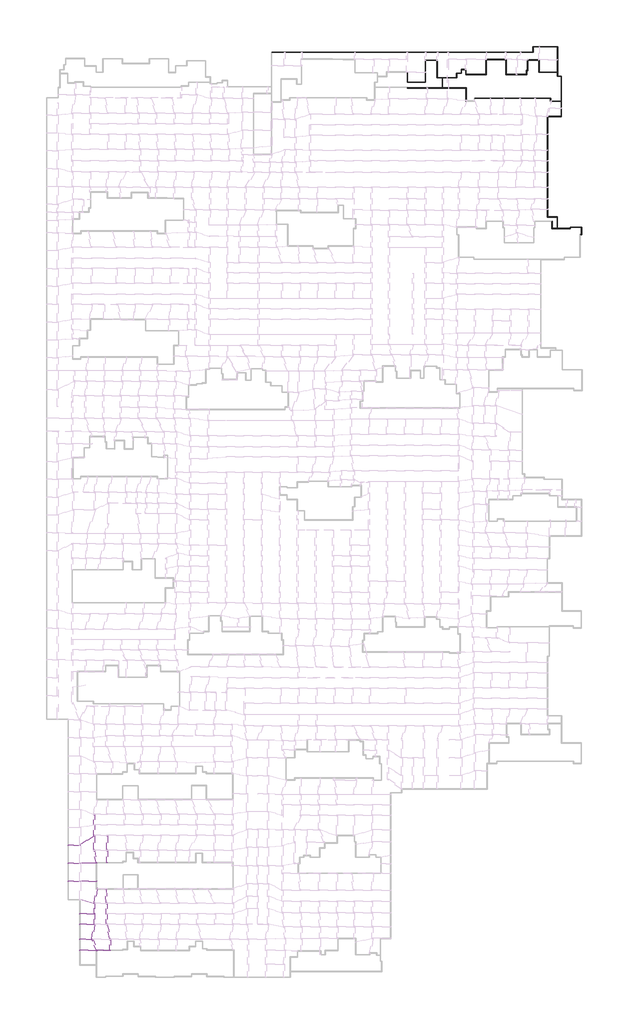
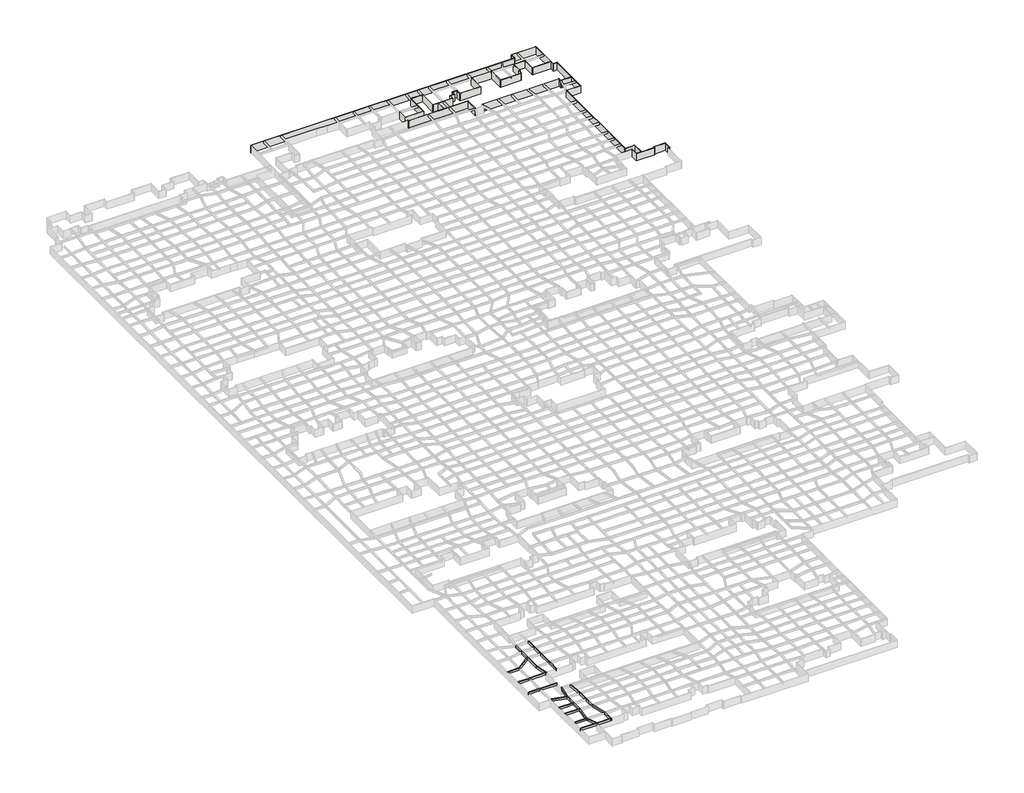
# One storey, part 10 of 45: 45 walls, 24 beams.
"""IFC4 building model written with IfcOpenShell, lengths in millimetres."""

from ifc_helpers import new_model, si_unit, frame, origin, origin_with_axes, place, context, project, spatial, polyline, outline, extrude, faceted_brep, element, save

model = new_model("IFC4")

# Units and contexts
model_context = context("Model", 3, world=origin())
ifc_project = project(units=[si_unit("LENGTHUNIT", "METRE", prefix="MILLI")], contexts=[model_context])

# Site, building, storey
site = spatial("IfcSite", under=ifc_project)
building = spatial("IfcBuilding", under=site)
storey = spatial("IfcBuildingStorey", under=building, Name="户型图", Elevation=0.0)

# Beams
placement = place(None, origin())
element("IfcBeam", 1, ObjectType="混凝土 - 矩形梁 : KL_beam", at=placement, inside=storey, context=model_context, shape_type="Brep", body=[
    faceted_brep([(-134129.6078212, -121175.3373066, 3300.0), (-134529.6078212, -121175.3373066, 3300.0), (-134529.6078212, -125381.8586454, 3300.0), (-134529.6078212, -125789.5105016, 3300.0), (-134529.6078212, -129967.4209018, 3300.0), (-134529.6078212, -130461.8480928, 3300.0), (-134529.6078212, -136482.7394466, 3300.0), (-134129.6078212, -136482.7394466, 3300.0), (-134129.6078212, -130269.3244435, 3300.0), (-134129.6078212, -129869.3244435, 3300.0), (-134129.6078212, -125746.3030805, 3300.0), (-134129.6078212, -125346.3030805, 3300.0), (-134529.6078212, -121175.3373066, 2500.0), (-134529.6078212, -125381.8586454, 2500.0), (-134529.6078212, -125789.5105016, 2500.0), (-134529.6078212, -129967.4209018, 2500.0), (-134529.6078212, -130461.8480928, 2500.0), (-134529.6078212, -136482.7394466, 2500.0), (-134129.6078212, -121175.3373066, 2500.0), (-134129.6078212, -125346.3030805, 2500.0), (-134129.6078212, -125746.3030805, 2500.0), (-134129.6078212, -129869.3244435, 2500.0), (-134129.6078212, -130269.3244435, 2500.0), (-134129.6078212, -136482.7394466, 2500.0)], [[[0, 1, 2, 3, 4, 5, 6, 7, 8, 9, 10, 11]], [[1, 12, 13, 14, 15, 16, 17, 6, 5, 4, 3, 2]], [[12, 18, 19, 20, 21, 22, 23, 17, 16, 15, 14, 13]], [[18, 0, 11, 10, 9, 8, 7, 23, 22, 21, 20, 19]], [[1, 0, 18, 12]], [[7, 6, 17, 23]]]),
])
element("IfcBeam", 2, ObjectType="混凝土 - 矩形梁 : KL_beam", at=placement, inside=storey, context=model_context, shape_type="SweptSolid", body=[
    extrude(outline(polyline([(-128929.6078212, -121175.3373066), (-128529.6078212, -121175.3373066), (-128529.6078212, -125346.3030805), (-128929.6078212, -125346.3030805), (-128929.6078212, -121175.3373066)])), frame((0.0, 0.0, 2500.0), z_axis=(0.0, 0.0, 1.0), x_axis=(1.0, 0.0, 0.0)), (0.0, 0.0, 1.0), 800.0),
    extrude(outline(polyline([(-128529.6078212, -136482.7394466), (-128929.6078212, -136482.7394466), (-128929.6078212, -130269.3244435), (-128529.6078212, -130269.3244435), (-128529.6078212, -136482.7394466)])), frame((0.0, 0.0, 2500.0), z_axis=(0.0, 0.0, 1.0), x_axis=(1.0, 0.0, 0.0)), (0.0, 0.0, 1.0), 800.0),
    extrude(outline(polyline([(-128929.6078212, -125746.3030805), (-128529.6078212, -125746.3030805), (-128529.6078212, -129869.3244435), (-128929.6078212, -129869.3244435), (-128929.6078212, -125746.3030805)])), frame((0.0, 0.0, 2500.0), z_axis=(0.0, 0.0, 1.0), x_axis=(1.0, 0.0, 0.0)), (0.0, 0.0, 1.0), 800.0),
])
element("IfcBeam", 3, ObjectType="混凝土 - 矩形梁 : KL_beam", at=placement, inside=storey, context=model_context, shape_type="SweptSolid", body=[
    extrude(outline(polyline([(-140235.0712547, -134607.1099192), (-140235.0712547, -134112.6827282), (-134529.6078212, -129967.4209018), (-134529.6078212, -130461.8480928), (-140235.0712547, -134607.1099192)])), frame((0.0, 0.0, 2500.0), z_axis=(0.0, 0.0, 1.0), x_axis=(1.0, 0.0, 0.0)), (0.0, 0.0, 1.0), 800.0),
])
element("IfcBeam", 4, ObjectType="混凝土 - 矩形梁 : KL_beam", at=placement, inside=storey, context=model_context, shape_type="SweptSolid", body=[
    extrude(outline(polyline([(-145640.2964556, -134705.27306), (-145640.2964556, -134305.27306), (-140635.0712547, -134305.27306), (-140635.0712547, -134705.27306), (-145640.2964556, -134705.27306)])), frame((0.0, 0.0, 2500.0), z_axis=(0.0, 0.0, 1.0), x_axis=(1.0, 0.0, 0.0)), (0.0, 0.0, 1.0), 800.0),
])
element("IfcBeam", 5, ObjectType="混凝土 - 矩形梁 : KL_beam", at=placement, inside=storey, context=model_context, shape_type="SweptSolid", body=[
    extrude(outline(polyline([(-128529.6078212, -142082.7394466), (-128929.6078212, -142082.7394466), (-128929.6078212, -136882.7394466), (-128529.6078212, -136882.7394466), (-128529.6078212, -142082.7394466)])), frame((0.0, 0.0, 2500.0), z_axis=(0.0, 0.0, 1.0), x_axis=(1.0, 0.0, 0.0)), (0.0, 0.0, 1.0), 800.0),
])
element("IfcBeam", 6, ObjectType="混凝土 - 矩形梁 : KL_beam", at=placement, inside=storey, context=model_context, shape_type="Brep", body=[
    faceted_brep([(-134086.4357741, -136882.7394466, 3300.0), (-134494.0876303, -136882.7394466, 3300.0), (-133510.465022, -141887.6116859, 3300.0), (-133432.3400776, -142285.1273204, 3300.0), (-133039.8483041, -142207.9897306, 3300.0), (-134494.0876303, -136882.7394466, 2500.0), (-133510.465022, -141887.6116859, 2500.0), (-133432.3400776, -142285.1273204, 2500.0), (-134086.4357741, -136882.7394466, 2500.0), (-133039.8483041, -142207.9897306, 2500.0)], [[[0, 1, 2, 3, 4]], [[3, 2, 1, 5, 6, 7]], [[7, 6, 5, 8, 9]], [[4, 9, 8, 0]], [[0, 8, 5, 1]], [[4, 3, 7, 9]]]),
])
element("IfcBeam", 7, ObjectType="混凝土 - 矩形梁 : KL_beam", at=placement, inside=storey, context=model_context, shape_type="SweptSolid", body=[
    extrude(outline(polyline([(-133510.465022, -141887.6116859), (-133432.3400776, -142285.1273204), (-140235.0712547, -142522.6839278), (-140235.0712547, -142122.4401101), (-133510.465022, -141887.6116859)])), frame((0.0, 0.0, 2500.0), z_axis=(0.0, 0.0, 1.0), x_axis=(1.0, 0.0, 0.0)), (0.0, 0.0, 1.0), 800.0),
])
element("IfcBeam", 8, ObjectType="混凝土 - 矩形梁 : KL_beam", at=placement, inside=storey, context=model_context, shape_type="SweptSolid", body=[
    extrude(outline(polyline([(-145635.2028364, -142529.5553627), (-145635.2028364, -142129.5553627), (-140635.0712547, -142129.5553627), (-140635.0712547, -142529.5553627), (-145635.2028364, -142529.5553627)])), frame((0.0, 0.0, 2500.0), z_axis=(0.0, 0.0, 1.0), x_axis=(1.0, 0.0, 0.0)), (0.0, 0.0, 1.0), 800.0),
])
element("IfcBeam", 9, ObjectType="混凝土 - 矩形梁 : KL_beam", at=placement, inside=storey, context=model_context, shape_type="SweptSolid", body=[
    extrude(outline(polyline([(-145640.2964556, -150329.5553627), (-145640.2964556, -149929.5553627), (-140635.0712547, -149929.5553627), (-140635.0712547, -150329.5553627), (-145640.2964556, -150329.5553627)])), frame((0.0, 0.0, 2500.0), z_axis=(0.0, 0.0, 1.0), x_axis=(1.0, 0.0, 0.0)), (0.0, 0.0, 1.0), 800.0),
])
element("IfcBeam", 10, ObjectType="混凝土 - 矩形梁 : KL_beam", at=placement, inside=storey, context=model_context, shape_type="SweptSolid", body=[
    extrude(outline(polyline([(-133235.6838551, -149929.5553627), (-133235.6838551, -150329.5553627), (-140235.0712547, -150329.5553627), (-140235.0712547, -149929.5553627), (-133235.6838551, -149929.5553627)])), frame((0.0, 0.0, 2500.0), z_axis=(0.0, 0.0, 1.0), x_axis=(1.0, 0.0, 0.0)), (0.0, 0.0, 1.0), 800.0),
])
element("IfcBeam", 11, ObjectType="混凝土 - 矩形梁 : KL_beam", at=placement, inside=storey, context=model_context, shape_type="Brep", body=[
    faceted_brep([(-134418.1629467, -159730.5423993, 3300.0), (-134018.1629467, -159765.5378647, 3300.0), (-133979.8122282, -159548.040132, 3300.0), (-132938.9946834, -153645.2705128, 3300.0), (-132868.4638912, -153245.2705128, 3300.0), (-133274.6345359, -153245.2705128, 3300.0), (-134378.1287333, -159503.4970927, 3300.0), (-134418.1629467, -159730.5423993, 2500.0), (-133274.6345359, -153245.2705128, 2500.0), (-134378.1287333, -159503.4970927, 2500.0), (-134018.1629467, -159765.5378647, 2500.0), (-132868.4638912, -153245.2705128, 2500.0), (-132938.9946834, -153645.2705128, 2500.0), (-133979.8122282, -159548.040132, 2500.0)], [[[0, 1, 2, 3, 4, 5, 6]], [[7, 0, 6, 5, 8, 9]], [[10, 7, 9, 8, 11, 12, 13]], [[1, 10, 13, 12, 11, 4, 3, 2]], [[1, 0, 7, 10]], [[5, 4, 11, 8]]]),
])
element("IfcBeam", 12, ObjectType="混凝土 - 矩形梁 : KL_beam", at=placement, inside=storey, context=model_context, shape_type="Brep", body=[
    faceted_brep([(-134018.1629467, -168962.0254944, 3300.0), (-134018.1629467, -168748.040132, 3300.0), (-134018.1629467, -164548.040132, 3300.0), (-134018.1629467, -164148.040132, 3300.0), (-134018.1629467, -159948.040132, 3300.0), (-134018.1629467, -159765.5378647, 3300.0), (-134418.1629467, -159730.5423993, 3300.0), (-134418.1629467, -159905.37019, 3300.0), (-134418.1629467, -164148.040132, 3300.0), (-134418.1629467, -164548.040132, 3300.0), (-134418.1629467, -168748.040132, 3300.0), (-134418.1629467, -168934.0547696, 3300.0), (-134418.1629467, -159730.5423993, 2500.0), (-134418.1629467, -159905.37019, 2500.0), (-134418.1629467, -164148.040132, 2500.0), (-134418.1629467, -164548.040132, 2500.0), (-134418.1629467, -168748.040132, 2500.0), (-134418.1629467, -168934.0547696, 2500.0), (-134018.1629467, -159765.5378647, 2500.0), (-134018.1629467, -159948.040132, 2500.0), (-134018.1629467, -164148.040132, 2500.0), (-134018.1629467, -164548.040132, 2500.0), (-134018.1629467, -168748.040132, 2500.0), (-134018.1629467, -168962.0254944, 2500.0)], [[[0, 1, 2, 3, 4, 5, 6, 7, 8, 9, 10, 11]], [[11, 10, 9, 8, 7, 6, 12, 13, 14, 15, 16, 17]], [[17, 16, 15, 14, 13, 12, 18, 19, 20, 21, 22, 23]], [[5, 4, 3, 2, 1, 0, 23, 22, 21, 20, 19, 18]], [[5, 18, 12, 6]], [[0, 11, 17, 23]]]),
])
element("IfcBeam", 13, ObjectType="混凝土 - 矩形梁 : KL_beam", at=placement, inside=storey, context=model_context, shape_type="Brep", body=[
    faceted_brep([(-134018.1629467, -168962.0254944, 3300.0), (-134418.1629467, -168934.0547696, 3300.0), (-134448.2366282, -169148.040132, 3300.0), (-135310.5627606, -175283.8093857, 3300.0), (-135342.4782502, -175510.8998937, 3300.0), (-135269.0825253, -175683.8093857, 3300.0), (-135039.0201973, -176225.8022656, 3300.0), (-134930.932576, -175456.7188778, 3300.0), (-134906.6317316, -175283.8093857, 3300.0), (-134044.3055992, -169148.040132, 3300.0), (-134418.1629467, -168934.0547696, 2500.0), (-134448.2366282, -169148.040132, 2500.0), (-135310.5627606, -175283.8093857, 2500.0), (-135342.4782502, -175510.8998937, 2500.0), (-134018.1629467, -168962.0254944, 2500.0), (-134044.3055992, -169148.040132, 2500.0), (-134906.6317316, -175283.8093857, 2500.0), (-134930.932576, -175456.7188778, 2500.0), (-135039.0201973, -176225.8022656, 2500.0), (-135269.0825253, -175683.8093857, 2500.0)], [[[0, 1, 2, 3, 4, 5, 6, 7, 8, 9]], [[1, 10, 11, 12, 13, 4, 3, 2]], [[10, 14, 15, 16, 17, 18, 19, 13, 12, 11]], [[14, 0, 9, 8, 7, 6, 18, 17, 16, 15]], [[0, 14, 10, 1]], [[6, 5, 4, 13, 19, 18]]]),
])
element("IfcBeam", 14, ObjectType="混凝土 - 矩形梁 : KL_beam", at=placement, inside=storey, context=model_context, shape_type="SweptSolid", body=[
    extrude(outline(polyline([(-128611.8494798, -159548.040132), (-129013.3774148, -159548.040132), (-129529.8028399, -153645.2705128), (-129128.2749049, -153645.2705128), (-128611.8494798, -159548.040132)])), frame((0.0, 0.0, 2500.0), z_axis=(0.0, 0.0, 1.0), x_axis=(1.0, 0.0, 0.0)), (0.0, 0.0, 1.0), 800.0),
])
element("IfcBeam", 15, ObjectType="混凝土 - 矩形梁 : KL_beam", at=placement, inside=storey, context=model_context, shape_type="Brep", body=[
    faceted_brep([(-128997.7870634, -168748.040132, 2500.0), (-128997.7870634, -168748.040132, 3300.0), (-128997.7870634, -164548.040132, 3300.0), (-128997.7870634, -164148.040132, 3300.0), (-128997.7870634, -159948.040132, 3300.0), (-128997.7870634, -159948.040132, 2500.0), (-128997.7870634, -164148.040132, 2500.0), (-128997.7870634, -164548.040132, 2500.0), (-128597.7870634, -168748.040132, 2500.0), (-128597.7870634, -168748.040132, 3300.0), (-128597.7870634, -159948.040132, 3300.0), (-128597.7870634, -159948.040132, 2500.0), (-128597.7870634, -164548.040132, 3300.0), (-128597.7870634, -164148.040132, 3300.0), (-128597.7870634, -164148.040132, 2500.0), (-128597.7870634, -164548.040132, 2500.0)], [[[0, 1, 2, 3, 4, 5, 6, 7]], [[1, 0, 8, 9]], [[10, 11, 5, 4]], [[10, 4, 3, 2, 1, 9, 12, 13]], [[5, 11, 14, 15, 8, 0, 7, 6]], [[11, 10, 13, 12, 9, 8, 15, 14]]]),
])
element("IfcBeam", 16, ObjectType="混凝土 - 矩形梁 : KL_beam", at=placement, inside=storey, context=model_context, shape_type="SweptSolid", body=[
    extrude(outline(polyline([(-127122.7494049, -175283.8093857), (-127533.271048, -175283.8093857), (-128949.8249968, -169148.040132), (-128539.3033537, -169148.040132), (-127122.7494049, -175283.8093857)])), frame((0.0, 0.0, 2500.0), z_axis=(0.0, 0.0, 1.0), x_axis=(1.0, 0.0, 0.0)), (0.0, 0.0, 1.0), 800.0),
])
element("IfcBeam", 17, ObjectType="混凝土 - 矩形梁 : KL_beam", at=placement, inside=storey, context=model_context, shape_type="Brep", body=[
    faceted_brep([(-127468.1198938, -180470.4346237, 2500.0), (-127468.1198938, -180470.4346237, 3300.0), (-127468.1198938, -180070.4346237, 3300.0), (-127468.1198938, -175683.8093857, 3300.0), (-127468.1198938, -175683.8093857, 2500.0), (-127468.1198938, -180070.4346237, 2500.0), (-127068.1198938, -175683.8093857, 3300.0), (-127068.1198938, -175683.8093857, 2500.0), (-127068.1198938, -180470.4346237, 3300.0), (-127068.1198938, -180470.4346237, 2500.0)], [[[0, 1, 2, 3, 4, 5]], [[6, 7, 4, 3]], [[6, 3, 2, 1, 8]], [[4, 7, 9, 0, 5]], [[7, 6, 8, 9]], [[8, 1, 0, 9]]]),
])
element("IfcBeam", 18, ObjectType="混凝土 - 矩形梁 : KL_beam", at=placement, inside=storey, context=model_context, shape_type="Brep", body=[
    faceted_brep([(-133237.2806572, -180470.4346237, 3300.0), (-132869.0787158, -180314.1421723, 3300.0), (-132972.5264327, -180070.4346237, 3300.0), (-134834.5383744, -175683.8093857, 3300.0), (-134930.932576, -175456.7188778, 3300.0), (-135039.0201973, -176225.8022656, 3300.0), (-133407.0705837, -180070.4346237, 3300.0), (-133237.2806572, -180470.4346237, 2500.0), (-135039.0201973, -176225.8022656, 2500.0), (-133407.0705837, -180070.4346237, 2500.0), (-132869.0787158, -180314.1421723, 2500.0), (-134930.932576, -175456.7188778, 2500.0), (-134834.5383744, -175683.8093857, 2500.0), (-132972.5264327, -180070.4346237, 2500.0)], [[[0, 1, 2, 3, 4, 5, 6]], [[7, 0, 6, 5, 8, 9]], [[10, 7, 9, 8, 11, 12, 13]], [[1, 10, 13, 12, 11, 4, 3, 2]], [[5, 4, 11, 8]], [[1, 0, 7, 10]]]),
])
element("IfcBeam", 19, ObjectType="混凝土 - 矩形梁 : KL_beam", at=placement, inside=storey, context=model_context, shape_type="SweptSolid", body=[
    extrude(outline(polyline([(-140540.1135348, -175683.8093857), (-140540.1135348, -175283.8093857), (-135310.5627606, -175283.8093857), (-135342.4782502, -175510.8998937), (-135269.0825253, -175683.8093857), (-140540.1135348, -175683.8093857)])), frame((0.0, 0.0, 2500.0), z_axis=(0.0, 0.0, 1.0), x_axis=(1.0, 0.0, 0.0)), (0.0, 0.0, 1.0), 800.0),
])
element("IfcBeam", 20, ObjectType="混凝土 - 矩形梁 : KL_beam", at=placement, inside=storey, context=model_context, shape_type="SweptSolid", body=[
    extrude(outline(polyline([(-140540.3423016, -169148.040132), (-140540.3423016, -168748.040132), (-134418.1629467, -168748.040132), (-134418.1629467, -168934.0547696), (-134448.2366282, -169148.040132), (-140540.3423016, -169148.040132)])), frame((0.0, 0.0, 2500.0), z_axis=(0.0, 0.0, 1.0), x_axis=(1.0, 0.0, 0.0)), (0.0, 0.0, 1.0), 800.0),
])
element("IfcBeam", 21, ObjectType="混凝土 - 矩形梁 : KL_beam", at=placement, inside=storey, context=model_context, shape_type="SweptSolid", body=[
    extrude(outline(polyline([(-140540.3423016, -164548.040132), (-140540.3423016, -164148.040132), (-134418.1629467, -164148.040132), (-134418.1629467, -164548.040132), (-140540.3423016, -164548.040132)])), frame((0.0, 0.0, 2500.0), z_axis=(0.0, 0.0, 1.0), x_axis=(1.0, 0.0, 0.0)), (0.0, 0.0, 1.0), 800.0),
])
element("IfcBeam", 22, ObjectType="混凝土 - 矩形梁 : KL_beam", at=placement, inside=storey, context=model_context, shape_type="SweptSolid", body=[
    extrude(outline(polyline([(-140235.0712547, -158496.0420414), (-140235.0712547, -158084.4694025), (-134378.1287333, -159503.4970927), (-134418.1629467, -159730.5423993), (-134418.1629467, -159905.37019), (-140235.0712547, -158496.0420414)])), frame((0.0, 0.0, 2500.0), z_axis=(0.0, 0.0, 1.0), x_axis=(1.0, 0.0, 0.0)), (0.0, 0.0, 1.0), 800.0),
])
element("IfcBeam", 23, ObjectType="混凝土 - 矩形梁 : KL_beam", at=placement, inside=storey, context=model_context, shape_type="SweptSolid", body=[
    extrude(outline(polyline([(-140540.2126007, -180470.4346237), (-140540.2126007, -180070.4346237), (-133407.0705837, -180070.4346237), (-133237.2806572, -180470.4346237), (-140540.2126007, -180470.4346237)])), frame((0.0, 0.0, 2500.0), z_axis=(0.0, 0.0, 1.0), x_axis=(1.0, 0.0, 0.0)), (0.0, 0.0, 1.0), 800.0),
])
element("IfcBeam", 24, ObjectType="混凝土 - 矩形梁 : KL_beam", at=placement, inside=storey, context=model_context, shape_type="SweptSolid", body=[
    extrude(outline(polyline([(-127468.1198938, -180470.4346237), (-133237.2806572, -180470.4346237), (-132869.0787158, -180314.1421723), (-132972.5264327, -180070.4346237), (-127468.1198938, -180070.4346237), (-127468.1198938, -180470.4346237)])), frame((0.0, 0.0, 2500.0), z_axis=(0.0, 0.0, 1.0), x_axis=(1.0, 0.0, 0.0)), (0.0, 0.0, 1.0), 800.0),
])

# Walls
element("IfcWall", 25, ObjectType="所有墙体", at=placement, inside=storey, context=model_context, shape_type="Brep", body=[
    faceted_brep([(77619.4783436, 131611.9876735, 0.0), (78319.4783436, 131611.9876735, 0.0), (78319.4783436, 131611.9876735, 3300.0), (77619.4783436, 131611.9876735, 3300.0), (77619.4783436, 131731.9876735, 0.0), (77619.4783436, 131731.9876735, 3300.0), (78199.4783436, 131731.9876735, 3300.0), (78319.4783436, 131731.9876735, 3300.0), (78319.4783436, 131731.9876735, 0.0), (78199.4783436, 131731.9876735, 0.0)], [[[0, 1, 2, 3]], [[4, 5, 6, 7, 8, 9]], [[1, 0, 4, 9, 8]], [[3, 2, 7, 6, 5]], [[0, 3, 5, 4]], [[2, 1, 8, 7]]]),
])
element("IfcWall", 26, ObjectType="所有墙体", at=placement, inside=storey, context=model_context, shape_type="Brep", body=[
    faceted_brep([(78319.4783436, 131731.9876735, 0.0), (78319.4783436, 134931.9876735, 0.0), (78319.4783436, 134931.9876735, 3300.0), (78319.4783436, 131731.9876735, 3300.0), (78199.4783436, 131731.9876735, 0.0), (78199.4783436, 131731.9876735, 3300.0), (78199.4783436, 134811.9876735, 3300.0), (78199.4783436, 134931.9876735, 3300.0), (78199.4783436, 134931.9876735, 0.0), (78199.4783436, 134811.9876735, 0.0)], [[[0, 1, 2, 3]], [[4, 5, 6, 7, 8, 9]], [[1, 0, 4, 9, 8]], [[3, 2, 7, 6, 5]], [[0, 3, 5, 4]], [[2, 1, 8, 7]]]),
])
element("IfcWall", 27, ObjectType="所有墙体", at=placement, inside=storey, context=model_context, shape_type="Brep", body=[
    faceted_brep([(78199.4783436, 134931.9876735, 0.0), (73299.4783436, 134931.9876735, 0.0), (73299.4783436, 134931.9876735, 3300.0), (78199.4783436, 134931.9876735, 3300.0), (78199.4783436, 134811.9876735, 0.0), (78199.4783436, 134811.9876735, 3300.0), (73419.4783436, 134811.9876735, 3300.0), (73299.4783436, 134811.9876735, 3300.0), (73299.4783436, 134811.9876735, 0.0), (73419.4783436, 134811.9876735, 0.0)], [[[0, 1, 2, 3]], [[4, 5, 6, 7, 8, 9]], [[1, 0, 4, 9, 8]], [[3, 2, 7, 6, 5]], [[0, 3, 5, 4]], [[2, 1, 8, 7]]]),
])
element("IfcWall", 28, ObjectType="所有墙体", at=placement, inside=storey, context=model_context, shape_type="Brep", body=[
    faceted_brep([(73299.4783436, 134811.9876735, 0.0), (73299.4783436, 134431.9876735, 0.0), (73299.4783436, 134311.9876735, 0.0), (73299.4783436, 134311.9876735, 3300.0), (73299.4783436, 134431.9876735, 3300.0), (73299.4783436, 134811.9876735, 3300.0), (73419.4783436, 134811.9876735, 0.0), (73419.4783436, 134811.9876735, 3300.0), (73419.4783436, 134311.9876735, 3300.0), (73419.4783436, 134311.9876735, 0.0)], [[[0, 1, 2, 3, 4, 5]], [[6, 7, 8, 9]], [[2, 1, 0, 6, 9]], [[5, 4, 3, 8, 7]], [[0, 5, 7, 6]], [[3, 2, 9, 8]]]),
])
element("IfcWall", 29, ObjectType="所有墙体", at=placement, inside=storey, context=model_context, shape_type="Brep", body=[
    faceted_brep([(73299.4783436, 134431.9876735, 0.0), (67719.4783436, 134431.9876735, 0.0), (67599.4783436, 134431.9876735, 0.0), (65419.4783436, 134431.9876735, 0.0), (65299.4783436, 134431.9876735, 0.0), (65299.4783436, 134431.9876735, 3300.0), (65419.4783436, 134431.9876735, 3300.0), (67599.4783436, 134431.9876735, 3300.0), (67719.4783436, 134431.9876735, 3300.0), (73299.4783436, 134431.9876735, 3300.0), (73299.4783436, 134311.9876735, 0.0), (73299.4783436, 134311.9876735, 3300.0), (65299.4783436, 134311.9876735, 3300.0), (65299.4783436, 134311.9876735, 0.0)], [[[0, 1, 2, 3, 4, 5, 6, 7, 8, 9]], [[10, 11, 12, 13]], [[4, 3, 2, 1, 0, 10, 13]], [[9, 8, 7, 6, 5, 12, 11]], [[0, 9, 11, 10]], [[5, 4, 13, 12]]]),
])
element("IfcWall", 30, ObjectType="所有墙体", at=placement, inside=storey, context=model_context, shape_type="Brep", body=[
    faceted_brep([(67719.4783436, 134431.9876735, 0.0), (67719.4783436, 139431.9876735, 0.0), (67719.4783436, 139431.9876735, 3300.0), (67719.4783436, 134431.9876735, 3300.0), (67599.4783436, 134431.9876735, 0.0), (67599.4783436, 134431.9876735, 3300.0), (67599.4783436, 139311.9876735, 3300.0), (67599.4783436, 139431.9876735, 3300.0), (67599.4783436, 139431.9876735, 0.0), (67599.4783436, 139311.9876735, 0.0)], [[[0, 1, 2, 3]], [[4, 5, 6, 7, 8, 9]], [[1, 0, 4, 9, 8]], [[3, 2, 7, 6, 5]], [[0, 3, 5, 4]], [[2, 1, 8, 7]]]),
])
element("IfcWall", 31, ObjectType="所有墙体", at=placement, inside=storey, context=model_context, shape_type="Brep", body=[
    faceted_brep([(67599.4783436, 139431.9876735, 0.0), (63519.4783436, 139431.9876735, 0.0), (63399.4783436, 139431.9876735, 0.0), (63399.4783436, 139431.9876735, 3300.0), (63519.4783436, 139431.9876735, 3300.0), (67599.4783436, 139431.9876735, 3300.0), (67599.4783436, 139311.9876735, 0.0), (67599.4783436, 139311.9876735, 3300.0), (63399.4783436, 139311.9876735, 3300.0), (63399.4783436, 139311.9876735, 0.0)], [[[0, 1, 2, 3, 4, 5]], [[6, 7, 8, 9]], [[2, 1, 0, 6, 9]], [[5, 4, 3, 8, 7]], [[0, 5, 7, 6]], [[3, 2, 9, 8]]]),
])
element("IfcWall", 32, ObjectType="所有墙体", at=placement, inside=storey, context=model_context, shape_type="Brep", body=[
    faceted_brep([(63519.4783436, 139431.9876735, 0.0), (63519.4783436, 183111.9876735, 0.0), (63519.4783436, 183231.9876735, 0.0), (63519.4783436, 183231.9876735, 3300.0), (63519.4783436, 183111.9876735, 3300.0), (63519.4783436, 139431.9876735, 3300.0), (63399.4783436, 139431.9876735, 0.0), (63399.4783436, 139431.9876735, 3300.0), (63399.4783436, 183231.9876735, 3300.0), (63399.4783436, 183231.9876735, 0.0)], [[[0, 1, 2, 3, 4, 5]], [[6, 7, 8, 9]], [[2, 1, 0, 6, 9]], [[5, 4, 3, 8, 7]], [[0, 5, 7, 6]], [[3, 2, 9, 8]]]),
])
element("IfcWall", 33, ObjectType="所有墙体", at=placement, inside=storey, context=model_context, shape_type="Brep", body=[
    faceted_brep([(63519.4783436, 183111.9876735, 0.0), (69519.4783436, 183111.9876735, 0.0), (69519.4783436, 183111.9876735, 3300.0), (63519.4783436, 183111.9876735, 3300.0), (63519.4783436, 183231.9876735, 0.0), (63519.4783436, 183231.9876735, 3300.0), (69399.4783436, 183231.9876735, 3300.0), (69519.4783436, 183231.9876735, 3300.0), (69519.4783436, 183231.9876735, 0.0), (69399.4783436, 183231.9876735, 0.0)], [[[0, 1, 2, 3]], [[4, 5, 6, 7, 8, 9]], [[1, 0, 4, 9, 8]], [[3, 2, 7, 6, 5]], [[0, 3, 5, 4]], [[2, 1, 8, 7]]]),
])
element("IfcWall", 34, ObjectType="所有墙体", at=placement, inside=storey, context=model_context, shape_type="Brep", body=[
    faceted_brep([(69519.4783436, 183231.9876735, 0.0), (69519.4783436, 200731.9876735, 0.0), (69519.4783436, 200731.9876735, 3300.0), (69519.4783436, 183231.9876735, 3300.0), (69399.4783436, 183231.9876735, 0.0), (69399.4783436, 183231.9876735, 3300.0), (69399.4783436, 189761.3641147, 3300.0), (69399.4783436, 189881.3641147, 3300.0), (69399.4783436, 200611.9876735, 3300.0), (69399.4783436, 200731.9876735, 3300.0), (69399.4783436, 200731.9876735, 0.0), (69399.4783436, 200611.9876735, 0.0), (69399.4783436, 189881.3641147, 0.0), (69399.4783436, 189761.3641147, 0.0)], [[[0, 1, 2, 3]], [[4, 5, 6, 7, 8, 9, 10, 11, 12, 13]], [[1, 0, 4, 13, 12, 11, 10]], [[3, 2, 9, 8, 7, 6, 5]], [[0, 3, 5, 4]], [[2, 1, 10, 9]]]),
])
element("IfcWall", 35, ObjectType="所有墙体", at=placement, inside=storey, context=model_context, shape_type="Brep", body=[
    faceted_brep([(69399.4783436, 200731.9876735, 0.0), (67819.4783436, 200731.9876735, 0.0), (67699.4783436, 200731.9876735, 0.0), (67699.4783436, 200731.9876735, 3300.0), (67819.4783436, 200731.9876735, 3300.0), (69399.4783436, 200731.9876735, 3300.0), (69399.4783436, 200611.9876735, 0.0), (69399.4783436, 200611.9876735, 3300.0), (67699.4783436, 200611.9876735, 3300.0), (67699.4783436, 200611.9876735, 0.0)], [[[0, 1, 2, 3, 4, 5]], [[6, 7, 8, 9]], [[2, 1, 0, 6, 9]], [[5, 4, 3, 8, 7]], [[0, 5, 7, 6]], [[3, 2, 9, 8]]]),
])
element("IfcWall", 36, ObjectType="所有墙体", at=placement, inside=storey, context=model_context, shape_type="Brep", body=[
    faceted_brep([(67819.4783436, 200731.9876735, 0.0), (67819.4783436, 213631.9876735, 0.0), (67819.4783436, 213631.9876735, 3300.0), (67819.4783436, 200731.9876735, 3300.0), (67699.4783436, 200731.9876735, 0.0), (67699.4783436, 200731.9876735, 3300.0), (67699.4783436, 202331.9680247, 3300.0), (67699.4783436, 202451.9680247, 3300.0), (67699.4783436, 213511.9876735, 3300.0), (67699.4783436, 213631.9876735, 3300.0), (67699.4783436, 213631.9876735, 0.0), (67699.4783436, 213511.9876735, 0.0), (67699.4783436, 202451.9680247, 0.0), (67699.4783436, 202331.9680247, 0.0)], [[[0, 1, 2, 3]], [[4, 5, 6, 7, 8, 9, 10, 11, 12, 13]], [[1, 0, 4, 13, 12, 11, 10]], [[3, 2, 9, 8, 7, 6, 5]], [[0, 3, 5, 4]], [[2, 1, 10, 9]]]),
])
element("IfcWall", 37, ObjectType="所有墙体", at=placement, inside=storey, context=model_context, shape_type="Brep", body=[
    faceted_brep([(67699.4783436, 213631.9876735, 0.0), (57099.4783436, 213631.9876735, 0.0), (57099.4783436, 213631.9876735, 3300.0), (67699.4783436, 213631.9876735, 3300.0), (67699.4783436, 213511.9876735, 0.0), (67699.4783436, 213511.9876735, 3300.0), (57219.4783436, 213511.9876735, 3300.0), (57099.4783436, 213511.9876735, 3300.0), (57099.4783436, 213511.9876735, 0.0), (57219.4783436, 213511.9876735, 0.0)], [[[0, 1, 2, 3]], [[4, 5, 6, 7, 8, 9]], [[1, 0, 4, 9, 8]], [[3, 2, 7, 6, 5]], [[0, 3, 5, 4]], [[2, 1, 8, 7]]]),
])
element("IfcWall", 38, ObjectType="所有墙体", at=placement, inside=storey, context=model_context, shape_type="Brep", body=[
    faceted_brep([(57099.4783436, 213511.9876735, 0.0), (57099.4783436, 211231.9876735, 0.0), (57099.4783436, 211111.9876735, 0.0), (57099.4783436, 211111.9876735, 3300.0), (57099.4783436, 211231.9876735, 3300.0), (57099.4783436, 213511.9876735, 3300.0), (57219.4783436, 213511.9876735, 0.0), (57219.4783436, 213511.9876735, 3300.0), (57219.4783436, 211111.9876735, 3300.0), (57219.4783436, 211111.9876735, 0.0)], [[[0, 1, 2, 3, 4, 5]], [[6, 7, 8, 9]], [[2, 1, 0, 6, 9]], [[5, 4, 3, 8, 7]], [[0, 5, 7, 6]], [[3, 2, 9, 8]]]),
])
element("IfcWall", 39, ObjectType="所有墙体", at=placement, inside=storey, context=model_context, shape_type="Brep", body=[
    faceted_brep([(57099.4783436, 211231.9876735, 0.0), (-57000.5216564, 211231.9876735, 0.0), (-57000.5216564, 211231.9876735, 3300.0), (57099.4783436, 211231.9876735, 3300.0), (57099.4783436, 211111.9876735, 0.0), (57099.4783436, 211111.9876735, 3300.0), (-56880.5216564, 211111.9876735, 3300.0), (-57000.5216564, 211111.9876735, 3300.0), (-57000.5216564, 211111.9876735, 0.0), (-56880.5216564, 211111.9876735, 0.0)], [[[0, 1, 2, 3]], [[4, 5, 6, 7, 8, 9]], [[1, 0, 4, 9, 8]], [[3, 2, 7, 6, 5]], [[0, 3, 5, 4]], [[2, 1, 8, 7]]]),
])
element("IfcWall", 40, ObjectType="所有墙体", at=placement, inside=storey, context=model_context, shape_type="Brep", body=[
    faceted_brep([(2251.0399311, 195871.9680247, 0.0), (2251.0399311, 195471.9680247, 0.0), (2251.0399311, 195471.9680247, 3300.0), (2251.0399311, 195871.9680247, 3300.0), (2371.0399311, 195871.9680247, 0.0), (2371.0399311, 195871.9680247, 3300.0), (2371.0399311, 195591.9680247, 3300.0), (2371.0399311, 195471.9680247, 3300.0), (2371.0399311, 195471.9680247, 0.0), (2371.0399311, 195591.9680247, 0.0)], [[[0, 1, 2, 3]], [[4, 5, 6, 7, 8, 9]], [[1, 0, 4, 9, 8]], [[3, 2, 7, 6, 5]], [[0, 3, 5, 4]], [[2, 1, 8, 7]]]),
])
element("IfcWall", 41, ObjectType="所有墙体", at=placement, inside=storey, context=model_context, shape_type="Brep", body=[
    faceted_brep([(2371.0399311, 195471.9680247, 0.0), (27851.0399311, 195471.9680247, 0.0), (27971.0399311, 195471.9680247, 0.0), (27971.0399311, 195471.9680247, 3300.0), (27851.0399311, 195471.9680247, 3300.0), (2371.0399311, 195471.9680247, 3300.0), (2371.0399311, 195591.9680247, 0.0), (2371.0399311, 195591.9680247, 3300.0), (17551.0399311, 195591.9680247, 3300.0), (17671.0399311, 195591.9680247, 3300.0), (27971.0399311, 195591.9680247, 3300.0), (27971.0399311, 195591.9680247, 0.0), (17671.0399311, 195591.9680247, 0.0), (17551.0399311, 195591.9680247, 0.0)], [[[0, 1, 2, 3, 4, 5]], [[6, 7, 8, 9, 10, 11, 12, 13]], [[2, 1, 0, 6, 13, 12, 11]], [[5, 4, 3, 10, 9, 8, 7]], [[0, 5, 7, 6]], [[3, 2, 11, 10]]]),
])
element("IfcWall", 42, ObjectType="所有墙体", at=placement, inside=storey, context=model_context, shape_type="Brep", body=[
    faceted_brep([(27851.0399311, 195471.9680247, 0.0), (27851.0399311, 189831.009409, 0.0), (27851.0399311, 189831.009409, 3300.0), (27851.0399311, 195471.9680247, 3300.0), (27971.0399311, 195471.9680247, 0.0), (27971.0399311, 195471.9680247, 3300.0), (27971.0399311, 189951.009409, 3300.0), (27971.0399311, 189831.009409, 3300.0), (27971.0399311, 189831.009409, 0.0), (27971.0399311, 189951.009409, 0.0)], [[[0, 1, 2, 3]], [[4, 5, 6, 7, 8, 9]], [[1, 0, 4, 9, 8]], [[3, 2, 7, 6, 5]], [[0, 3, 5, 4]], [[2, 1, 8, 7]]]),
])
element("IfcWall", 43, ObjectType="所有墙体", at=placement, inside=storey, context=model_context, shape_type="Brep", body=[
    faceted_brep([(31556.641355, 191031.009409, 0.0), (64736.641355, 191031.009409, 0.0), (64856.641355, 191031.009409, 0.0), (64856.641355, 191031.009409, 3300.0), (64736.641355, 191031.009409, 3300.0), (31556.641355, 191031.009409, 3300.0), (31556.641355, 191151.009409, 0.0), (31556.641355, 191151.009409, 3300.0), (64856.641355, 191151.009409, 3300.0), (64856.641355, 191151.009409, 0.0)], [[[0, 1, 2, 3, 4, 5]], [[6, 7, 8, 9]], [[2, 1, 0, 6, 9]], [[5, 4, 3, 8, 7]], [[0, 5, 7, 6]], [[3, 2, 9, 8]]]),
])
element("IfcWall", 44, ObjectType="所有墙体", at=placement, inside=storey, context=model_context, shape_type="Brep", body=[
    faceted_brep([(64736.641355, 191031.009409, 0.0), (64736.641355, 189761.3641147, 0.0), (64736.641355, 189761.3641147, 3300.0), (64736.641355, 191031.009409, 3300.0), (64856.641355, 191031.009409, 0.0), (64856.641355, 191031.009409, 3300.0), (64856.641355, 189881.3641147, 3300.0), (64856.641355, 189761.3641147, 3300.0), (64856.641355, 189761.3641147, 0.0), (64856.641355, 189881.3641147, 0.0)], [[[0, 1, 2, 3]], [[4, 5, 6, 7, 8, 9]], [[1, 0, 4, 9, 8]], [[3, 2, 7, 6, 5]], [[0, 3, 5, 4]], [[2, 1, 8, 7]]]),
])
element("IfcWall", 45, ObjectType="所有墙体", at=placement, inside=storey, context=model_context, shape_type="SweptSolid", body=[
    extrude(outline(polyline([(69399.4783436, 189761.3641147), (64856.641355, 189761.3641147), (64856.641355, 189881.3641147), (69399.4783436, 189881.3641147), (69399.4783436, 189761.3641147)])), origin_with_axes(), (0.0, 0.0, 1.0), 3300.0),
])
element("IfcWall", 46, ObjectType="所有墙体", at=placement, inside=storey, context=model_context, shape_type="Brep", body=[
    faceted_brep([(2251.0399311, 198031.9680247, 0.0), (10271.0399311, 198031.9680247, 0.0), (10271.0399311, 198031.9680247, 3300.0), (2251.0399311, 198031.9680247, 3300.0), (2251.0399311, 198151.9680247, 0.0), (2251.0399311, 198151.9680247, 3300.0), (2371.0399311, 198151.9680247, 3300.0), (10151.0399311, 198151.9680247, 3300.0), (10271.0399311, 198151.9680247, 3300.0), (10271.0399311, 198151.9680247, 0.0), (10151.0399311, 198151.9680247, 0.0), (2371.0399311, 198151.9680247, 0.0)], [[[0, 1, 2, 3]], [[4, 5, 6, 7, 8, 9, 10, 11]], [[1, 0, 4, 11, 10, 9]], [[3, 2, 8, 7, 6, 5]], [[2, 1, 9, 8]], [[0, 3, 5, 4]]]),
])
element("IfcWall", 47, ObjectType="所有墙体", at=placement, inside=storey, context=model_context, shape_type="Brep", body=[
    faceted_brep([(10271.0399311, 198151.9680247, 0.0), (10271.0399311, 207631.9680247, 0.0), (10271.0399311, 207751.9680247, 0.0), (10271.0399311, 207751.9680247, 3300.0), (10271.0399311, 207631.9680247, 3300.0), (10271.0399311, 198151.9680247, 3300.0), (10151.0399311, 198151.9680247, 0.0), (10151.0399311, 198151.9680247, 3300.0), (10151.0399311, 207751.9680247, 3300.0), (10151.0399311, 207751.9680247, 0.0)], [[[0, 1, 2, 3, 4, 5]], [[6, 7, 8, 9]], [[2, 1, 0, 6, 9]], [[5, 4, 3, 8, 7]], [[0, 5, 7, 6]], [[3, 2, 9, 8]]]),
])
element("IfcWall", 48, ObjectType="所有墙体", at=placement, inside=storey, context=model_context, shape_type="Brep", body=[
    faceted_brep([(10271.0399311, 207631.9680247, 0.0), (15251.0399311, 207631.9680247, 0.0), (15371.0399311, 207631.9680247, 0.0), (15371.0399311, 207631.9680247, 3300.0), (15251.0399311, 207631.9680247, 3300.0), (10271.0399311, 207631.9680247, 3300.0), (10271.0399311, 207751.9680247, 0.0), (10271.0399311, 207751.9680247, 3300.0), (15371.0399311, 207751.9680247, 3300.0), (15371.0399311, 207751.9680247, 0.0)], [[[0, 1, 2, 3, 4, 5]], [[6, 7, 8, 9]], [[2, 1, 0, 6, 9]], [[5, 4, 3, 8, 7]], [[0, 5, 7, 6]], [[3, 2, 9, 8]]]),
])
element("IfcWall", 49, ObjectType="所有墙体", at=placement, inside=storey, context=model_context, shape_type="Brep", body=[
    faceted_brep([(15251.0399311, 207631.9680247, 0.0), (15251.0399311, 199931.9680247, 0.0), (15251.0399311, 199931.9680247, 3300.0), (15251.0399311, 207631.9680247, 3300.0), (15371.0399311, 207631.9680247, 0.0), (15371.0399311, 207631.9680247, 3300.0), (15371.0399311, 200051.9680247, 3300.0), (15371.0399311, 199931.9680247, 3300.0), (15371.0399311, 199931.9680247, 0.0), (15371.0399311, 200051.9680247, 0.0)], [[[0, 1, 2, 3]], [[4, 5, 6, 7, 8, 9]], [[1, 0, 4, 9, 8]], [[3, 2, 7, 6, 5]], [[0, 3, 5, 4]], [[2, 1, 8, 7]]]),
])
element("IfcWall", 50, ObjectType="所有墙体", at=placement, inside=storey, context=model_context, shape_type="Brep", body=[
    faceted_brep([(15371.0399311, 199931.9680247, 0.0), (17551.0399311, 199931.9680247, 0.0), (17671.0399311, 199931.9680247, 0.0), (23871.0399311, 199931.9680247, 0.0), (23871.0399311, 199931.9680247, 3300.0), (17671.0399311, 199931.9680247, 3300.0), (17551.0399311, 199931.9680247, 3300.0), (15371.0399311, 199931.9680247, 3300.0), (15371.0399311, 200051.9680247, 0.0), (15371.0399311, 200051.9680247, 3300.0), (23751.0399311, 200051.9680247, 3300.0), (23871.0399311, 200051.9680247, 3300.0), (23871.0399311, 200051.9680247, 0.0), (23751.0399311, 200051.9680247, 0.0)], [[[0, 1, 2, 3, 4, 5, 6, 7]], [[8, 9, 10, 11, 12, 13]], [[3, 2, 1, 0, 8, 13, 12]], [[7, 6, 5, 4, 11, 10, 9]], [[0, 7, 9, 8]], [[4, 3, 12, 11]]]),
])
element("IfcWall", 51, ObjectType="所有墙体", at=placement, inside=storey, context=model_context, shape_type="SweptSolid", body=[
    extrude(outline(polyline([(17551.0399311, 195591.9680247), (17551.0399311, 199931.9680247), (17671.0399311, 199931.9680247), (17671.0399311, 195591.9680247), (17551.0399311, 195591.9680247)])), origin_with_axes(), (0.0, 0.0, 1.0), 3300.0),
])
element("IfcWall", 52, ObjectType="所有墙体", at=placement, inside=storey, context=model_context, shape_type="Brep", body=[
    faceted_brep([(23871.0399311, 200051.9680247, 0.0), (23871.0399311, 201931.9680247, 0.0), (23871.0399311, 202051.9680247, 0.0), (23871.0399311, 202051.9680247, 3300.0), (23871.0399311, 201931.9680247, 3300.0), (23871.0399311, 200051.9680247, 3300.0), (23751.0399311, 200051.9680247, 0.0), (23751.0399311, 200051.9680247, 3300.0), (23751.0399311, 202051.9680247, 3300.0), (23751.0399311, 202051.9680247, 0.0)], [[[0, 1, 2, 3, 4, 5]], [[6, 7, 8, 9]], [[2, 1, 0, 6, 9]], [[5, 4, 3, 8, 7]], [[0, 5, 7, 6]], [[3, 2, 9, 8]]]),
])
element("IfcWall", 53, ObjectType="所有墙体", at=placement, inside=storey, context=model_context, shape_type="Brep", body=[
    faceted_brep([(23871.0399311, 201931.9680247, 0.0), (25871.0399311, 201931.9680247, 0.0), (25871.0399311, 201931.9680247, 3300.0), (23871.0399311, 201931.9680247, 3300.0), (23871.0399311, 202051.9680247, 0.0), (23871.0399311, 202051.9680247, 3300.0), (25751.0399311, 202051.9680247, 3300.0), (25871.0399311, 202051.9680247, 3300.0), (25871.0399311, 202051.9680247, 0.0), (25751.0399311, 202051.9680247, 0.0)], [[[0, 1, 2, 3]], [[4, 5, 6, 7, 8, 9]], [[1, 0, 4, 9, 8]], [[3, 2, 7, 6, 5]], [[0, 3, 5, 4]], [[2, 1, 8, 7]]]),
])
element("IfcWall", 54, ObjectType="所有墙体", at=placement, inside=storey, context=model_context, shape_type="Brep", body=[
    faceted_brep([(25871.0399311, 202051.9680247, 0.0), (25871.0399311, 203531.9680247, 0.0), (25871.0399311, 203651.9680247, 0.0), (25871.0399311, 203651.9680247, 3300.0), (25871.0399311, 203531.9680247, 3300.0), (25871.0399311, 202051.9680247, 3300.0), (25751.0399311, 202051.9680247, 0.0), (25751.0399311, 202051.9680247, 3300.0), (25751.0399311, 203651.9680247, 3300.0), (25751.0399311, 203651.9680247, 0.0)], [[[0, 1, 2, 3, 4, 5]], [[6, 7, 8, 9]], [[2, 1, 0, 6, 9]], [[5, 4, 3, 8, 7]], [[0, 5, 7, 6]], [[3, 2, 9, 8]]]),
])
element("IfcWall", 55, ObjectType="所有墙体", at=placement, inside=storey, context=model_context, shape_type="Brep", body=[
    faceted_brep([(25871.0399311, 203531.9680247, 0.0), (27775.6474887, 203531.9680247, 0.0), (27895.6474887, 203531.9680247, 0.0), (27895.6474887, 203531.9680247, 3300.0), (27775.6474887, 203531.9680247, 3300.0), (25871.0399311, 203531.9680247, 3300.0), (25871.0399311, 203651.9680247, 0.0), (25871.0399311, 203651.9680247, 3300.0), (27895.6474887, 203651.9680247, 3300.0), (27895.6474887, 203651.9680247, 0.0)], [[[0, 1, 2, 3, 4, 5]], [[6, 7, 8, 9]], [[2, 1, 0, 6, 9]], [[5, 4, 3, 8, 7]], [[0, 5, 7, 6]], [[3, 2, 9, 8]]]),
])
element("IfcWall", 56, ObjectType="所有墙体", at=placement, inside=storey, context=model_context, shape_type="Brep", body=[
    faceted_brep([(27775.6474887, 203531.9680247, 0.0), (27775.6474887, 201331.9680247, 0.0), (27775.6474887, 201331.9680247, 3300.0), (27775.6474887, 203531.9680247, 3300.0), (27895.6474887, 203531.9680247, 0.0), (27895.6474887, 203531.9680247, 3300.0), (27895.6474887, 201451.9680247, 3300.0), (27895.6474887, 201331.9680247, 3300.0), (27895.6474887, 201331.9680247, 0.0), (27895.6474887, 201451.9680247, 0.0)], [[[0, 1, 2, 3]], [[4, 5, 6, 7, 8, 9]], [[1, 0, 4, 9, 8]], [[3, 2, 7, 6, 5]], [[0, 3, 5, 4]], [[2, 1, 8, 7]]]),
])
element("IfcWall", 57, ObjectType="所有墙体", at=placement, inside=storey, context=model_context, shape_type="Brep", body=[
    faceted_brep([(27895.6474887, 201331.9680247, 0.0), (36695.6474887, 201331.9680247, 0.0), (36695.6474887, 201331.9680247, 3300.0), (27895.6474887, 201331.9680247, 3300.0), (27895.6474887, 201451.9680247, 0.0), (27895.6474887, 201451.9680247, 3300.0), (36575.6474887, 201451.9680247, 3300.0), (36695.6474887, 201451.9680247, 3300.0), (36695.6474887, 201451.9680247, 0.0), (36575.6474887, 201451.9680247, 0.0)], [[[0, 1, 2, 3]], [[4, 5, 6, 7, 8, 9]], [[1, 0, 4, 9, 8]], [[3, 2, 7, 6, 5]], [[0, 3, 5, 4]], [[2, 1, 8, 7]]]),
])
element("IfcWall", 58, ObjectType="所有墙体", at=placement, inside=storey, context=model_context, shape_type="Brep", body=[
    faceted_brep([(36695.6474887, 201451.9680247, 0.0), (36695.6474887, 207951.9876735, 0.0), (36695.6474887, 208071.9876735, 0.0), (36695.6474887, 208071.9876735, 3300.0), (36695.6474887, 207951.9876735, 3300.0), (36695.6474887, 201451.9680247, 3300.0), (36575.6474887, 201451.9680247, 0.0), (36575.6474887, 201451.9680247, 3300.0), (36575.6474887, 208071.9876735, 3300.0), (36575.6474887, 208071.9876735, 0.0)], [[[0, 1, 2, 3, 4, 5]], [[6, 7, 8, 9]], [[2, 1, 0, 6, 9]], [[5, 4, 3, 8, 7]], [[0, 5, 7, 6]], [[3, 2, 9, 8]]]),
])
element("IfcWall", 59, ObjectType="所有墙体", at=placement, inside=storey, context=model_context, shape_type="Brep", body=[
    faceted_brep([(36695.6474887, 207951.9876735, 0.0), (45275.6474887, 207951.9876735, 0.0), (45395.6474887, 207951.9876735, 0.0), (45395.6474887, 207951.9876735, 3300.0), (45275.6474887, 207951.9876735, 3300.0), (36695.6474887, 207951.9876735, 3300.0), (36695.6474887, 208071.9876735, 0.0), (36695.6474887, 208071.9876735, 3300.0), (45395.6474887, 208071.9876735, 3300.0), (45395.6474887, 208071.9876735, 0.0)], [[[0, 1, 2, 3, 4, 5]], [[6, 7, 8, 9]], [[2, 1, 0, 6, 9]], [[5, 4, 3, 8, 7]], [[0, 5, 7, 6]], [[3, 2, 9, 8]]]),
])
element("IfcWall", 60, ObjectType="所有墙体", at=placement, inside=storey, context=model_context, shape_type="Brep", body=[
    faceted_brep([(45275.6474887, 207951.9876735, 0.0), (45275.6474887, 201331.9680247, 0.0), (45275.6474887, 201331.9680247, 3300.0), (45275.6474887, 207951.9876735, 3300.0), (45395.6474887, 207951.9876735, 0.0), (45395.6474887, 207951.9876735, 3300.0), (45395.6474887, 201451.9680247, 3300.0), (45395.6474887, 201331.9680247, 3300.0), (45395.6474887, 201331.9680247, 0.0), (45395.6474887, 201451.9680247, 0.0)], [[[0, 1, 2, 3]], [[4, 5, 6, 7, 8, 9]], [[1, 0, 4, 9, 8]], [[3, 2, 7, 6, 5]], [[0, 3, 5, 4]], [[2, 1, 8, 7]]]),
])
element("IfcWall", 61, ObjectType="所有墙体", at=placement, inside=storey, context=model_context, shape_type="Brep", body=[
    faceted_brep([(45395.6474887, 201331.9680247, 0.0), (54395.6474887, 201331.9680247, 0.0), (54395.6474887, 201331.9680247, 3300.0), (45395.6474887, 201331.9680247, 3300.0), (45395.6474887, 201451.9680247, 0.0), (45395.6474887, 201451.9680247, 3300.0), (54275.6474887, 201451.9680247, 3300.0), (54395.6474887, 201451.9680247, 3300.0), (54395.6474887, 201451.9680247, 0.0), (54275.6474887, 201451.9680247, 0.0)], [[[0, 1, 2, 3]], [[4, 5, 6, 7, 8, 9]], [[1, 0, 4, 9, 8]], [[3, 2, 7, 6, 5]], [[0, 3, 5, 4]], [[2, 1, 8, 7]]]),
])
element("IfcWall", 62, ObjectType="所有墙体", at=placement, inside=storey, context=model_context, shape_type="Brep", body=[
    faceted_brep([(54395.6474887, 201451.9680247, 0.0), (54395.6474887, 203131.9680247, 0.0), (54395.6474887, 203251.9680247, 0.0), (54395.6474887, 203251.9680247, 3300.0), (54395.6474887, 203131.9680247, 3300.0), (54395.6474887, 201451.9680247, 3300.0), (54275.6474887, 201451.9680247, 0.0), (54275.6474887, 201451.9680247, 3300.0), (54275.6474887, 203251.9680247, 3300.0), (54275.6474887, 203251.9680247, 0.0)], [[[0, 1, 2, 3, 4, 5]], [[6, 7, 8, 9]], [[2, 1, 0, 6, 9]], [[5, 4, 3, 8, 7]], [[0, 5, 7, 6]], [[3, 2, 9, 8]]]),
])
element("IfcWall", 63, ObjectType="所有墙体", at=placement, inside=storey, context=model_context, shape_type="Brep", body=[
    faceted_brep([(54395.6474887, 203131.9680247, 0.0), (54795.6474887, 203131.9680247, 0.0), (54795.6474887, 203131.9680247, 3300.0), (54395.6474887, 203131.9680247, 3300.0), (54395.6474887, 203251.9680247, 0.0), (54395.6474887, 203251.9680247, 3300.0), (54675.6474887, 203251.9680247, 3300.0), (54795.6474887, 203251.9680247, 3300.0), (54795.6474887, 203251.9680247, 0.0), (54675.6474887, 203251.9680247, 0.0)], [[[0, 1, 2, 3]], [[4, 5, 6, 7, 8, 9]], [[1, 0, 4, 9, 8]], [[3, 2, 7, 6, 5]], [[0, 3, 5, 4]], [[2, 1, 8, 7]]]),
])
element("IfcWall", 64, ObjectType="所有墙体", at=placement, inside=storey, context=model_context, shape_type="Brep", body=[
    faceted_brep([(54795.6474887, 203251.9680247, 0.0), (54795.6474887, 207731.9680247, 0.0), (54795.6474887, 207851.9680247, 0.0), (54795.6474887, 207851.9680247, 3300.0), (54795.6474887, 207731.9680247, 3300.0), (54795.6474887, 203251.9680247, 3300.0), (54675.6474887, 203251.9680247, 0.0), (54675.6474887, 203251.9680247, 3300.0), (54675.6474887, 207851.9680247, 3300.0), (54675.6474887, 207851.9680247, 0.0)], [[[0, 1, 2, 3, 4, 5]], [[6, 7, 8, 9]], [[2, 1, 0, 6, 9]], [[5, 4, 3, 8, 7]], [[0, 5, 7, 6]], [[3, 2, 9, 8]]]),
])
element("IfcWall", 65, ObjectType="所有墙体", at=placement, inside=storey, context=model_context, shape_type="Brep", body=[
    faceted_brep([(54795.6474887, 207731.9680247, 0.0), (59675.6474887, 207731.9680247, 0.0), (59795.6474887, 207731.9680247, 0.0), (59795.6474887, 207731.9680247, 3300.0), (59675.6474887, 207731.9680247, 3300.0), (54795.6474887, 207731.9680247, 3300.0), (54795.6474887, 207851.9680247, 0.0), (54795.6474887, 207851.9680247, 3300.0), (59795.6474887, 207851.9680247, 3300.0), (59795.6474887, 207851.9680247, 0.0)], [[[0, 1, 2, 3, 4, 5]], [[6, 7, 8, 9]], [[2, 1, 0, 6, 9]], [[5, 4, 3, 8, 7]], [[0, 5, 7, 6]], [[3, 2, 9, 8]]]),
])
element("IfcWall", 66, ObjectType="所有墙体", at=placement, inside=storey, context=model_context, shape_type="Brep", body=[
    faceted_brep([(59675.6474887, 207731.9680247, 0.0), (59675.6474887, 202331.9680247, 0.0), (59675.6474887, 202331.9680247, 3300.0), (59675.6474887, 207731.9680247, 3300.0), (59795.6474887, 207731.9680247, 0.0), (59795.6474887, 207731.9680247, 3300.0), (59795.6474887, 202451.9680247, 3300.0), (59795.6474887, 202331.9680247, 3300.0), (59795.6474887, 202331.9680247, 0.0), (59795.6474887, 202451.9680247, 0.0)], [[[0, 1, 2, 3]], [[4, 5, 6, 7, 8, 9]], [[1, 0, 4, 9, 8]], [[3, 2, 7, 6, 5]], [[0, 3, 5, 4]], [[2, 1, 8, 7]]]),
])
element("IfcWall", 67, ObjectType="所有墙体", at=placement, inside=storey, context=model_context, shape_type="SweptSolid", body=[
    extrude(outline(polyline([(67699.4783436, 202331.9680247), (59795.6474887, 202331.9680247), (59795.6474887, 202451.9680247), (67699.4783436, 202451.9680247), (67699.4783436, 202331.9680247)])), origin_with_axes(), (0.0, 0.0, 1.0), 3300.0),
])
element("IfcWall", 68, ObjectType="所有墙体", at=placement, inside=storey, context=model_context, shape_type="Brep", body=[
    faceted_brep([(2371.0399311, 198151.9680247, 0.0), (2371.0399311, 202651.9680247, 0.0), (2371.0399311, 202651.9680247, 3300.0), (2371.0399311, 198151.9680247, 3300.0), (2251.0399311, 198151.9680247, 0.0), (2251.0399311, 198151.9680247, 3300.0), (2251.0399311, 202531.9680247, 3300.0), (2251.0399311, 202651.9680247, 3300.0), (2251.0399311, 202651.9680247, 0.0), (2251.0399311, 202531.9680247, 0.0)], [[[0, 1, 2, 3]], [[4, 5, 6, 7, 8, 9]], [[1, 0, 4, 9, 8]], [[3, 2, 7, 6, 5]], [[0, 3, 5, 4]], [[2, 1, 8, 7]]]),
])
element("IfcWall", 69, ObjectType="所有墙体", at=placement, inside=storey, context=model_context, shape_type="Brep", body=[
    faceted_brep([(65419.4783436, 134431.9876735, 0.0), (65419.4783436, 137531.9876735, 0.0), (65419.4783436, 137531.9876735, 3300.0), (65419.4783436, 134431.9876735, 3300.0), (65299.4783436, 134431.9876735, 0.0), (65299.4783436, 134431.9876735, 3300.0), (65299.4783436, 137411.9876735, 3300.0), (65299.4783436, 137531.9876735, 3300.0), (65299.4783436, 137531.9876735, 0.0), (65299.4783436, 137411.9876735, 0.0)], [[[0, 1, 2, 3]], [[4, 5, 6, 7, 8, 9]], [[1, 0, 4, 9, 8]], [[3, 2, 7, 6, 5]], [[0, 3, 5, 4]], [[2, 1, 8, 7]]]),
])

save(model, "model.ifc")

# Revit data of these elements
# Type "混凝土 - 矩形梁 : KL_beam"
#   Length [instance default] = 1524 mm
#   b = 400 mm
#   h = 800 mm
#   Structural Material [instance default] = 混凝土 - 现场浇注混凝土
#   Assembly Code = ""
# Type "所有墙体"
#   Layers, outside or top first: 120 mm "默认" (function 1)
# Elements 1, 2, 3, 4, 5, 6, 7, 8, 9, 10, 11, 12, 13, 14, 15, 16, 17, 18, 19, 20, 21, 22, 23, 24 (IfcBeam, "混凝土 - 矩形梁 : KL_beam")
#   Comments = ""
#   Structural Material = none
#   Phase Created = 新构造
# Elements 25, 26, 27, 28, 29, 30, 31, 32, 33, 34, 35, 36, 37, 38, 39, 40, 41, 42, 43, 44, 45, 46, 47, 48, 49, 50, 51, 52, 53, 54, 55, 56, 57, 58, 59, 60, 61, 62, 63, 64, 65, 66, 67, 68, 69 (IfcWall, "所有墙体")
#   Top Offset = 0 mm
#   Base Offset = 0 mm
#   wall height = 3300 mm
#   Phase Created = 新构造
#   Base Constraint = 户型图
#   Top Constraint = 层高
#   Materials on its faces: "默认"
# Materials
#   "混凝土 - 现场浇注混凝土": class "混凝土", colour RGB 192 192 192, transparency 0
#   "默认": class "其他", colour RGB 192 192 192, transparency 0, Cost = 0
